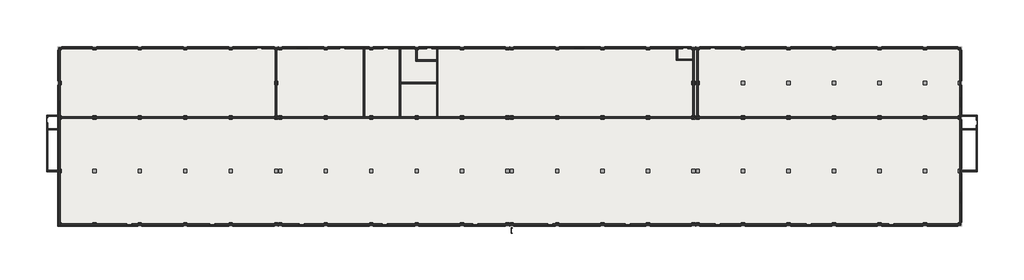
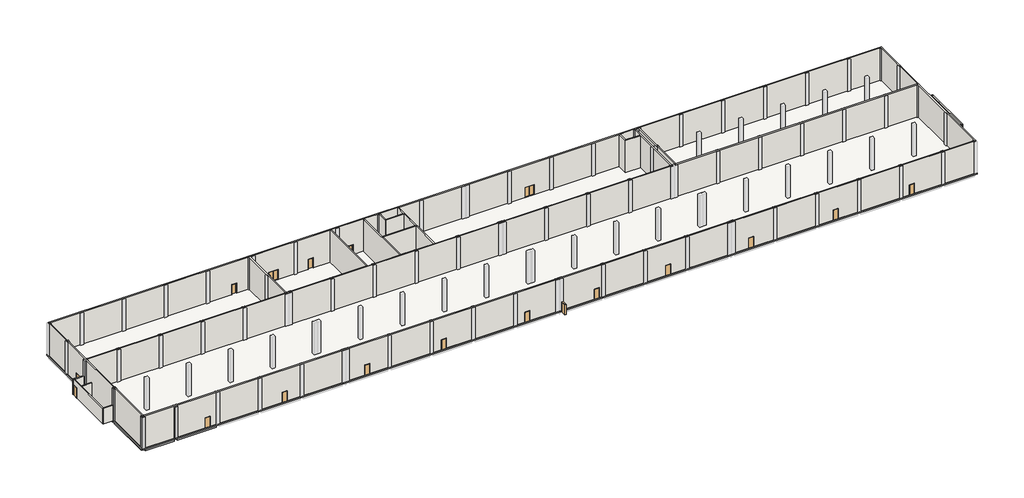
# One storey, part 1 of 4: 27 walls, 24 doors, 4 beams, 4 columns, 1 slab.
# Revit data of these elements (continued)
# Project information
#   H_Seismic Condition = "A as per ASCE 7-10"
#   H_Soil Condition = "C as per ASCE 7-10"
#   H_Basic Wind Speed = "58.3m/s ASCE7-10"
#   H_DS Project Code = "FAASA2302"
#   H_Project Abbreviation = "SACE2"
#   H_Project Division = "화공"
#   H_Project Finish = "2027-03-05"
#   H_Project Location = "Jafurah, Saudi Arabia"
#   H_Project Start = "2024-01-03"
#   H_Project Type = "EPC"
#   H_Smart Code = "FAASA2302"
#   Project Issue Date = "Issue Date"
#   Project Status = "Project Status"
#   Client Name = "Owner"
#   Project Address = "Enter address here"
#   Project Name = "Project Name"
#   Project Number = "0001"
# Grids (mm)
#   "X20": line (127180, 11877.337) -> (127180, -38909.79)
#   "Y3": line (-7812.06, -6000.479) -> (162922.774, -6000.479)
#   "X3": line (10130, 11877.337) -> (10130, -38909.79)
#   "X5": line (26530, 11877.337) -> (26530, -38909.79)
#   "X6": line (34730, 11877.337) -> (34730, -38909.79)
#   "X7": line (35480, 11877.337) -> (35480, -38909.79)
#   "X8": line (43680, 11877.337) -> (43680, -38909.79)
#   "X9": line (51880, 11877.337) -> (51880, -38909.79)
#   "X10": line (60080, 11877.337) -> (60080, -38909.79)
#   "X11": line (68280, 11877.337) -> (68280, -38909.79)
#   "X12": line (76480, 11877.337) -> (76480, -38909.79)
#   "X13": line (77230, 11877.337) -> (77230, -38909.79)
#   "X14": line (85430, 11877.337) -> (85430, -38909.79)
#   "X15": line (93630, 11877.337) -> (93630, -38909.79)
#   "X16": line (101830, 11877.337) -> (101830, -38909.79)
#   "X17": line (110030, 11877.337) -> (110030, -38909.79)
#   "X18": line (110780, 11877.337) -> (110780, -38909.79)
#   "X19": line (118980, 11877.337) -> (118980, -38909.79)
#   "X21": line (135380, 11877.337) -> (135380, -38909.79)
#   "X22": line (143580, 11877.337) -> (143580, -38909.79)
#   "X24": line (158130, 11877.337) -> (158130, -38909.79)
#   "Y2": line (-7812.06, 249.521) -> (162922.774, 249.521)
#   "X1": line (-4370, 11877.337) -> (-4370, -38909.79)
#   "X2": line (1930, 11877.337) -> (1930, -38909.79)
#   "Y1": line (-7812.06, 6499.521) -> (162922.774, 6499.521)
#   "X23": line (151780, 11877.337) -> (151780, -38909.79)
#   "Y4": line (-7812.06, -15650.479) -> (162922.774, -15650.479)
#   "Y5": line (-7812.06, -25300.479) -> (162922.774, -25300.479)
#   "X4": line (18330, 11877.337) -> (18330, -38909.79)
# Type "RC Beam_Rectangular : H_SB_AR_S16_TG_B400xH600"
#   중앙부 하부근 = ""
#   중앙부 상부근 = ""
#   중앙부 보조근 = ""
#   중앙부 늑근 = ""
#   외단부 하부근 = ""
#   외단부 상부근 = ""
#   외단부 보조근 = ""
#   외단부 늑근 = ""
#   부호 = "TG2"
#   내단부 하부근 = ""
#   내단부 상부근 = ""
#   내단부 보조근 = ""
#   내단부 늑근 = ""
#   ALL 하부근 = "3-D20"
#   ALL 상부근 = "4-D20"
#   ALL 보조근 = ""
#   ALL 늑근 = "2-D10 @120"
#   Width = 350 mm
#   Height = 600 mm
#   Length [instance default] = 1524 mm
#   b = 350 mm
#   h = 600 mm
#   hec_material3 [instance default] = none
#   hec_material2 [instance default] = none
#   hec_material1 [instance default] = none
#   Structural Material [instance default] = none
#   Assembly Code = ""
# Type "RC_Column_Rectangular : H_SC_AR_S15_W600xL600"
#   Width = 600 mm
#   Length = 600 mm
#   hec_material3 [instance default] = none
#   hec_material2 [instance default] = none
#   hec_material1 [instance default] = none
#   Structural Material [instance default] = none
#   Description = (empty or 0)
# Type "Double Door_Steel : H_DR_AR_B12_Double Door_Steel_W2000xH2100"
#   Type Mark = ""
#   프레임 = ""
#   철물 = ""
#   유리/마감 = ""
#   위치/개소 = ""
#   부호 = "1/SD"
#   문번호 = ""
#   문기호 = "SD"
#   Analytic Construction = "<None>"
#   Height = 2100 mm
#   Width = 1800 mm
#   Define Thermal Properties by = 1
#   문 틀 = none
#   문 = none
#   Function = (empty or 0)
#   Assembly Code = ""
#   Wall Closure = (empty or 0)
# Type "Single Door_Steel : H_DR_AR_B12_Single Door_Steel_W1000xH2100"
#   Type Mark = "SD"
#   Analytic Construction = "<None>"
#   프레임 투영 외부. = 25 mm
#   프레임 투영 내부. = 25 mm
#   프레임 폭 = 75 mm
#   Height = 2100 mm
#   Width = 1000 mm
#   Define Thermal Properties by = 1
#   문 패널 = none
#   문 프레임 = none
#   Function = (empty or 0)
#   Wall Closure = (empty or 0)
# Type "H_FL_AR_S17_RC Slab T150"
#   Keynote = ""
#   Type Comments = ""
#   Description = ""
#   Function = 1
#   Layers, outside or top first: 150 mm no material (function 1)
# Type "H_WA_AR_B02_Ext Wall_RC T200"
#   Type Comments = ""
#   Layers, outside or top first: 0 mm no material (function 100); 0 mm no material (function 100); 200 mm no material (function 1); 0 mm no material (function 100); 0 mm no material (function 100); 0 mm no material (function 100)
# Type "H_WA_AR_B02_Int Wall_Block T200"
#   Type Comments = ""
#   Layers, outside or top first: 0 mm no material (function 100); 12 mm no material (function 2); 200 mm no material (function 1); 12 mm no material (function 2); 10 mm no material (function 5)
# Elements 1, 2, 3, 4 (IfcBeam, "RC Beam_Rectangular : H_SB_AR_S16_TG_B400xH600")
#   Comments = ""
#   hec_material3 = none
#   hec_material2 = none
#   hec_material1 = none
#   Structural Material = none
#   Phase Created = New Construction
# Elements 5, 6, 7, 8 (IfcColumn, "RC_Column_Rectangular : H_SC_AR_S15_W600xL600")
#   Comments = ""
#   hec_material3 = none
#   hec_material2 = none
#   hec_material1 = none
#   Structural Material = none
#   Phase Created = New Construction
# Elements 9, 10, 11, 12, 13 (IfcDoor, "Double Door_Steel : H_DR_AR_B12_Double Door_Steel_W2000xH2100")
#   Phase Created = New Construction
# Elements 14, 15, 16, 17, 18, 19, 20, 21, 22, 23, 24, 25, 26, 27, 28, 29, 30, 31, 32 (IfcDoor, "Single Door_Steel : H_DR_AR_B12_Single Door_Steel_W1000xH2100")
#   Phase Created = New Construction
# Element 33 (IfcSlab, "H_FL_AR_S17_RC Slab T150")
#   Height Offset From Level = 0 mm
#   Phase Created = New Construction
#   Materials on its faces: "Default Floor"
# Elements 34, 35, 36, 58 (IfcWall, "H_WA_AR_B02_Ext Wall_RC T200")
#   Top Offset = 0 mm
#   Base Offset = 0 mm
#   wall height = 6650 mm
#   Phase Created = New Construction
#   Base Constraint = 01_T.O.F
#   Top Constraint = 03_T.O.C_1
#   Materials on its faces: "Default Wall"
# Elements 37, 38, 39, 40, 41, 42, 43, 47, 48, 49, 50, 51, 52, 53, 54 (IfcWall, "H_WA_AR_B02_Int Wall_Block T200")
#   Top Offset = 0 mm
#   Base Offset = 0 mm
#   wall height = 6650 mm
#   Phase Created = New Construction
#   Base Constraint = 01_T.O.F
#   Top Constraint = 03_T.O.C_1
#   Materials on its faces: "Default Wall"
# Elements 44, 45, 46, 55, 56, 57, 59, 60 (IfcWall, "H_WA_AR_B02_Ext Wall_RC T200")
#   Top Offset = 0 mm
#   Base Offset = 0 mm
#   wall height = 3150 mm
#   Phase Created = New Construction
#   Base Constraint = 01_T.O.F
#   Top Constraint = 02_T.O.LOWROOF
#   Materials on its faces: "Default Wall"
# Materials
#   "Default Floor": class "Miscellaneous", colour RGB 80 80 80, transparency 0
#   "Default Wall": class "Miscellaneous", colour RGB 80 80 80, transparency 0
